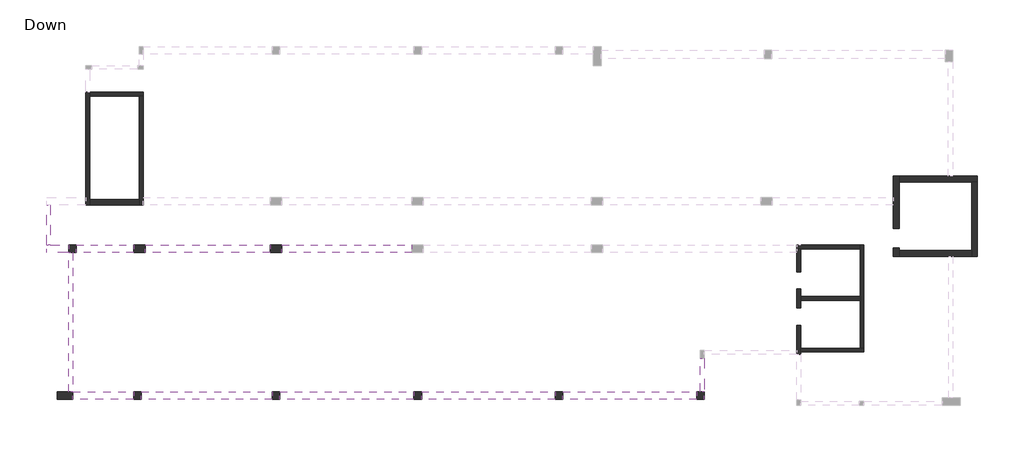
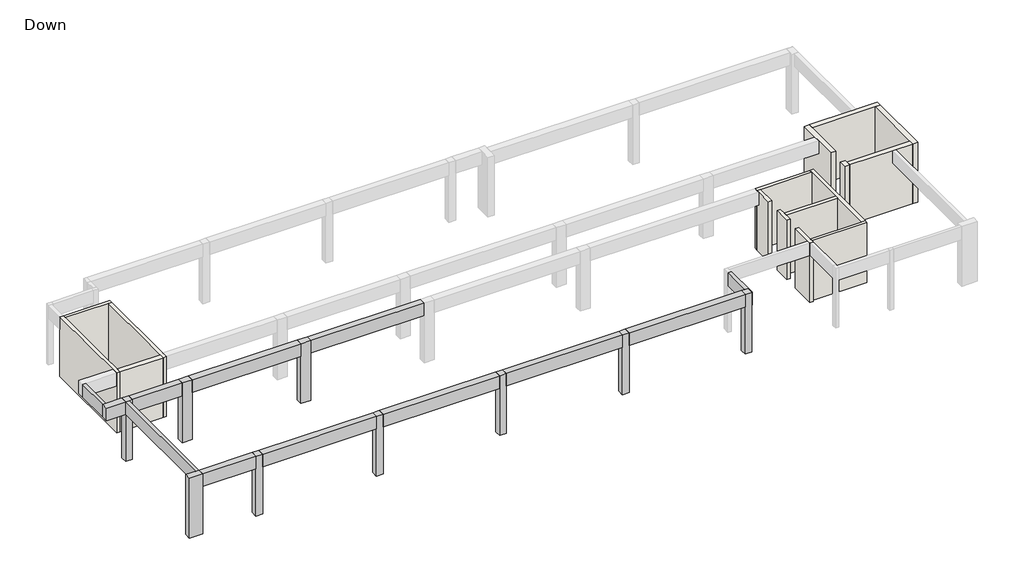
# One storey, part 1 of 2: 16 walls, 12 beams, 9 columns.
"""IFC4 building model written with IfcOpenShell, lengths in millimetres."""

from ifc_helpers import new_model, si_unit, frame, origin, origin_with_axes, place, context, project, spatial, polyline, outline, extrude, faceted_brep, element, save

model = new_model("IFC4")

# Units and contexts
model_context = context("Model", 3, world=origin())
ifc_project = project(units=[si_unit("LENGTHUNIT", "METRE", prefix="MILLI")], contexts=[model_context])

# Site, building, storey
site = spatial("IfcSite", under=ifc_project)
building = spatial("IfcBuilding", under=site)
storey = spatial("IfcBuildingStorey", under=building, Name="Down", Elevation=0.0)

# Beams
placement = place(None, origin())
element("IfcBeam", 1, ObjectType="Concrete Rectengular Beam : 20/80", at=placement, inside=storey, context=model_context, shape_type="Brep", body=[
    faceted_brep([(15342.1345122, -9540.2012066, 3800.0), (15342.1345122, -9940.2012066, 3800.0), (15344.7363769, -9940.2012066, 3800.0), (15344.7363769, -7771.4322554, 3800.0), (15144.7363769, -7771.4322554, 3800.0), (15144.7363769, -9540.2012066, 3800.0), (15144.7363769, -7771.4322554, 3520.0), (15144.7363769, -7771.4322554, 3000.0), (15144.7363769, -9540.2012066, 3000.0), (15144.7363769, -9540.2012066, 3520.0), (15342.1345122, -9940.2012066, 3000.0), (15342.1345122, -9540.2012066, 3000.0), (15344.7363769, -7771.4322554, 3000.0), (15344.7363769, -9940.2012066, 3000.0)], [[[0, 1, 2, 3, 4, 5]], [[5, 4, 6, 7, 8, 9]], [[10, 11, 8, 7, 12, 13]], [[12, 3, 2, 13]], [[0, 11, 10, 1]], [[11, 0, 5, 9, 8]], [[4, 3, 12, 7, 6]], [[13, 2, 1, 10]]]),
])
element("IfcBeam", 2, ObjectType="Concrete Rectengular Beam : 20/80", at=placement, inside=storey, context=model_context, shape_type="Brep", body=[
    faceted_brep([(-17707.5957255, -2249.6811448, 3800.0), (-17907.5957255, -2249.6811448, 3800.0), (-17907.5957255, -9540.2012066, 3800.0), (-17707.5957255, -9540.2012066, 3800.0), (-17907.5957255, -2249.6811448, 3000.0), (-17907.5957255, -9540.2012066, 3000.0), (-17707.5957255, -2249.6811448, 3000.0), (-17707.5957255, -9540.2012066, 3000.0), (-17707.5957255, -2249.6811448, 3520.0), (-17707.5957255, -9540.2012066, 3520.0)], [[[0, 1, 2, 3]], [[1, 4, 5, 2]], [[4, 6, 7, 5]], [[6, 8, 0, 3, 9, 7]], [[1, 0, 8, 6, 4]], [[3, 2, 5, 7, 9]]]),
])
element("IfcBeam", 3, ObjectType="Concrete Rectengular Beam : 20/80", at=placement, inside=storey, context=model_context, shape_type="Brep", body=[
    faceted_brep([(-18867.5920656, 245.3255739, 3800.0), (-19067.5920656, 245.3255739, 3800.0), (-19067.5920656, -1849.6811448, 3800.0), (-18867.5920656, -1849.6811448, 3800.0), (-18867.5920656, 245.3255739, 3000.0), (-18867.5920656, 245.3255739, 3520.0), (-18867.5920656, -1849.6811448, 3520.0), (-18867.5920656, -1849.6811448, 3000.0), (-19067.5920656, 245.3255739, 3000.0), (-19067.5920656, -1849.6811448, 3000.0)], [[[0, 1, 2, 3]], [[4, 5, 0, 3, 6, 7]], [[8, 4, 7, 9]], [[1, 8, 9, 2]], [[1, 0, 5, 4, 8]], [[3, 2, 9, 7, 6]]]),
])
element("IfcBeam", 4, ObjectType="Concrete Rectengular Beam : 40/80", at=placement, inside=storey, context=model_context, shape_type="SweptSolid", body=[
    extrude(outline(polyline([(7948.8072182, -9940.2012066), (7948.8072182, -9540.2012066), (14942.1345122, -9540.2012066), (14942.1345122, -9940.2012066), (7948.8072182, -9940.2012066)])), frame((0.0, 0.0, 3000.0), z_axis=(0.0, 0.0, 1.0), x_axis=(1.0, 0.0, 0.0)), (0.0, 0.0, 1.0), 800.0),
])
element("IfcBeam", 5, ObjectType="Concrete Rectengular Beam : 40/80", at=placement, inside=storey, context=model_context, shape_type="SweptSolid", body=[
    extrude(outline(polyline([(551.39348, -9940.2012066), (551.39348, -9540.2012066), (7548.8072182, -9540.2012066), (7548.8072182, -9940.2012066), (551.39348, -9940.2012066)])), frame((0.0, 0.0, 3000.0), z_axis=(0.0, 0.0, 1.0), x_axis=(1.0, 0.0, 0.0)), (0.0, 0.0, 1.0), 800.0),
])
element("IfcBeam", 6, ObjectType="Concrete Rectengular Beam : 40/80", at=placement, inside=storey, context=model_context, shape_type="SweptSolid", body=[
    extrude(outline(polyline([(-6857.9830653, -9940.2012066), (-6857.9830653, -9540.2012066), (151.39348, -9540.2012066), (151.39348, -9940.2012066), (-6857.9830653, -9940.2012066)])), frame((0.0, 0.0, 3000.0), z_axis=(0.0, 0.0, 1.0), x_axis=(1.0, 0.0, 0.0)), (0.0, 0.0, 1.0), 800.0),
])
element("IfcBeam", 7, ObjectType="Concrete Rectengular Beam : 40/80", at=placement, inside=storey, context=model_context, shape_type="SweptSolid", body=[
    extrude(outline(polyline([(-14112.2396142, -9940.2012066), (-14112.2396142, -9540.2012066), (-7257.9830653, -9540.2012066), (-7257.9830653, -9940.2012066), (-14112.2396142, -9940.2012066)])), frame((0.0, 0.0, 3000.0), z_axis=(0.0, 0.0, 1.0), x_axis=(1.0, 0.0, 0.0)), (0.0, 0.0, 1.0), 800.0),
])
element("IfcBeam", 8, ObjectType="Concrete Rectengular Beam : 40/80", at=placement, inside=storey, context=model_context, shape_type="Brep", body=[
    faceted_brep([(-14512.2396142, -9940.2012066, 3800.0), (-14512.2396142, -9540.2012066, 3800.0), (-17707.5957255, -9540.2012066, 3800.0), (-17707.5957255, -9940.2012066, 3800.0), (-14512.2396142, -9540.2012066, 3000.0), (-17707.5957255, -9540.2012066, 3000.0), (-17707.5957255, -9540.2012066, 3520.0), (-14512.2396142, -9940.2012066, 3000.0), (-17707.5957255, -9940.2012066, 3000.0)], [[[0, 1, 2, 3]], [[1, 4, 5, 6, 2]], [[4, 7, 8, 5]], [[7, 0, 3, 8]], [[1, 0, 7, 4]], [[3, 2, 6, 5, 8]]]),
])
element("IfcBeam", 9, ObjectType="Concrete Rectengular Beam : 40/80", at=placement, inside=storey, context=model_context, shape_type="SweptSolid", body=[
    extrude(outline(polyline([(-2249.6811448, 3000.0), (-2249.6811448, 3800.0), (-1851.1339506, 3800.0), (-1851.1339506, 3520.0), (-1849.6811448, 3520.0), (-1849.6811448, 3000.0), (-2249.6811448, 3000.0)])), frame((-17507.5957255, 0.0, 0.0), z_axis=(1.0, 0.0, 0.0), x_axis=(0.0, 1.0, 0.0)), (0.0, 0.0, 1.0), 2997.9865781),
])
element("IfcBeam", 10, ObjectType="Concrete Rectengular Beam : 40/80", at=placement, inside=storey, context=model_context, shape_type="SweptSolid", body=[
    extrude(outline(polyline([(-2249.6811448, 3000.0), (-2249.6811448, 3800.0), (-1851.1339506, 3800.0), (-1851.1339506, 3520.0), (-1849.6811448, 3520.0), (-1849.6811448, 3000.0), (-2249.6811448, 3000.0)])), frame((-13909.6091474, 0.0, 0.0), z_axis=(1.0, 0.0, 0.0), x_axis=(0.0, 1.0, 0.0)), (0.0, 0.0, 1.0), 6551.6260822),
])
element("IfcBeam", 11, ObjectType="Concrete Rectengular Beam : 40/80", at=placement, inside=storey, context=model_context, shape_type="SweptSolid", body=[
    extrude(outline(polyline([(-2249.6811448, 3000.0), (-2249.6811448, 3800.0), (-1851.1339506, 3800.0), (-1851.1339506, 3520.0), (-1849.6811448, 3520.0), (-1849.6811448, 3000.0), (-2249.6811448, 3000.0)])), frame((-6757.9830653, 0.0, 0.0), z_axis=(1.0, 0.0, 0.0), x_axis=(0.0, 1.0, 0.0)), (0.0, 0.0, 1.0), 6809.3765453),
])
element("IfcBeam", 12, ObjectType="Concrete Rectengular Beam : 40/80", at=placement, inside=storey, context=model_context, shape_type="Brep", body=[
    faceted_brep([(-19067.5920656, -1849.6811448, 3800.0), (-19067.5920656, -2249.6811448, 3800.0), (-17907.5957255, -2249.6811448, 3800.0), (-17907.5957255, -1851.1339506, 3800.0), (-18867.5920656, -1851.1339506, 3800.0), (-18867.5920656, -1849.6811448, 3800.0), (-19067.5920656, -1849.6811448, 3000.0), (-18867.5920656, -1849.6811448, 3520.0), (-17907.5957255, -1849.6811448, 3520.0), (-17907.5957255, -1849.6811448, 3000.0), (-18867.5920656, -1849.6811448, 3000.0), (-17907.5957255, -2249.6811448, 3000.0), (-19067.5920656, -2249.6811448, 3000.0), (-17907.5957255, -1851.1339506, 3520.0), (-18867.5920656, -1851.1339506, 3520.0)], [[[0, 1, 2, 3, 4, 5]], [[6, 0, 5, 7, 8, 9, 10]], [[9, 11, 12, 6, 10]], [[11, 2, 1, 12]], [[2, 11, 9, 8, 13, 3]], [[1, 0, 6, 12]], [[7, 14, 13, 8]], [[14, 4, 3, 13]], [[4, 14, 7, 5]]]),
])

# Columns
element("IfcColumn", 13, ObjectType="Concrete Rectengular Column : 40/40", at=placement, inside=storey, context=model_context, shape_type="Brep", body=[
    faceted_brep([(-17507.5957255, -1849.6811448, 0.0), (-17507.5957255, -2249.6811448, 0.0), (-17907.5957255, -2249.6811448, 0.0), (-17907.5957255, -1849.6811448, 0.0), (-17507.5957255, -1849.6811448, 3800.0), (-17507.5957255, -1851.1339506, 3800.0), (-17507.5957255, -2249.6811448, 3800.0), (-17507.5957255, -1849.6811448, 3520.0), (-17707.5957255, -2249.6811448, 3800.0), (-17907.5957255, -2249.6811448, 3800.0), (-17907.5957255, -1851.1339506, 3800.0), (-17907.5957255, -1849.6811448, 3800.0), (-17907.5957255, -1849.6811448, 3520.0)], [[[0, 1, 2, 3]], [[4, 5, 6, 1, 0, 7]], [[6, 8, 9, 2, 1]], [[9, 10, 11, 12, 3, 2]], [[11, 4, 7, 0, 3, 12]], [[4, 11, 10, 9, 8, 6, 5]]]),
])
element("IfcColumn", 14, ObjectType="Concrete Rectengular Column : 40/40", at=placement, inside=storey, context=model_context, shape_type="SweptSolid", body=[
    extrude(outline(polyline([(-14112.2396142, -9540.2012066), (-14112.2396142, -9940.2012066), (-14512.2396142, -9940.2012066), (-14512.2396142, -9540.2012066), (-14112.2396142, -9540.2012066)])), origin_with_axes(), (0.0, 0.0, 1.0), 3800.0),
])
element("IfcColumn", 15, ObjectType="Concrete Rectengular Column : 40/40", at=placement, inside=storey, context=model_context, shape_type="SweptSolid", body=[
    extrude(outline(polyline([(-6857.9830653, -9540.2012066), (-6857.9830653, -9940.2012066), (-7257.9830653, -9940.2012066), (-7257.9830653, -9540.2012066), (-6857.9830653, -9540.2012066)])), origin_with_axes(), (0.0, 0.0, 1.0), 3800.0),
])
element("IfcColumn", 16, ObjectType="Concrete Rectengular Column : 40/40", at=placement, inside=storey, context=model_context, shape_type="SweptSolid", body=[
    extrude(outline(polyline([(551.39348, -9540.2012066), (551.39348, -9940.2012066), (151.39348, -9940.2012066), (151.39348, -9540.2012066), (551.39348, -9540.2012066)])), origin_with_axes(), (0.0, 0.0, 1.0), 3800.0),
])
element("IfcColumn", 17, ObjectType="Concrete Rectengular Column : 40/40", at=placement, inside=storey, context=model_context, shape_type="SweptSolid", body=[
    extrude(outline(polyline([(7948.8072182, -9540.2012066), (7948.8072182, -9940.2012066), (7548.8072182, -9940.2012066), (7548.8072182, -9540.2012066), (7948.8072182, -9540.2012066)])), origin_with_axes(), (0.0, 0.0, 1.0), 3800.0),
])
element("IfcColumn", 18, ObjectType="Concrete Rectengular Column : 40/40", at=placement, inside=storey, context=model_context, shape_type="Brep", body=[
    faceted_brep([(15342.1345122, -9540.2012066, 0.0), (15342.1345122, -9940.2012066, 0.0), (14942.1345122, -9940.2012066, 0.0), (14942.1345122, -9540.2012066, 0.0), (15342.1345122, -9540.2012066, 3800.0), (15342.1345122, -9940.2012066, 3800.0), (14942.1345122, -9940.2012066, 3800.0), (14942.1345122, -9540.2012066, 3800.0), (15144.7363769, -9540.2012066, 3800.0)], [[[0, 1, 2, 3]], [[4, 5, 1, 0]], [[5, 6, 2, 1]], [[6, 7, 3, 2]], [[7, 8, 4, 0, 3]], [[4, 8, 7, 6, 5]]]),
])
element("IfcColumn", 19, ObjectType="Concrete Rectengular Column : 40/60", at=placement, inside=storey, context=model_context, shape_type="Brep", body=[
    faceted_brep([(-14509.6091474, -1849.6811448, 0.0), (-13909.6091474, -1849.6811448, 0.0), (-13909.6091474, -2249.6811448, 0.0), (-14509.6091474, -2249.6811448, 0.0), (-14509.6091474, -1849.6811448, 3800.0), (-13909.6091474, -1849.6811448, 3800.0), (-13909.6091474, -1849.6811448, 3520.0), (-14509.6091474, -1849.6811448, 3520.0), (-13909.6091474, -1851.1339506, 3800.0), (-13909.6091474, -2249.6811448, 3800.0), (-14509.6091474, -2249.6811448, 3800.0), (-14509.6091474, -1851.1339506, 3800.0)], [[[0, 1, 2, 3]], [[4, 5, 6, 1, 0, 7]], [[5, 8, 9, 2, 1, 6]], [[9, 10, 3, 2]], [[10, 11, 4, 7, 0, 3]], [[4, 11, 10, 9, 8, 5]]]),
])
element("IfcColumn", 20, ObjectType="Concrete Rectengular Column : 40/60", at=placement, inside=storey, context=model_context, shape_type="Brep", body=[
    faceted_brep([(-7357.9830653, -1849.6811448, 0.0), (-6757.9830653, -1849.6811448, 0.0), (-6757.9830653, -2249.6811448, 0.0), (-7357.9830653, -2249.6811448, 0.0), (-7357.9830653, -1849.6811448, 3800.0), (-6757.9830653, -1849.6811448, 3800.0), (-6757.9830653, -1849.6811448, 3520.0), (-7357.9830653, -1849.6811448, 3520.0), (-6757.9830653, -1851.1339506, 3800.0), (-6757.9830653, -2249.6811448, 3800.0), (-7357.9830653, -2249.6811448, 3800.0), (-7357.9830653, -1851.1339506, 3800.0)], [[[0, 1, 2, 3]], [[4, 5, 6, 1, 0, 7]], [[5, 8, 9, 2, 1, 6]], [[9, 10, 3, 2]], [[10, 11, 4, 7, 0, 3]], [[4, 11, 10, 9, 8, 5]]]),
])
element("IfcColumn", 21, ObjectType="Concrete Rectengular Column : 40/80", at=placement, inside=storey, context=model_context, shape_type="SweptSolid", body=[
    extrude(outline(polyline([(-18507.5957255, -9540.2012066), (-17707.5957255, -9540.2012066), (-17707.5957255, -9940.2012066), (-18507.5957255, -9940.2012066), (-18507.5957255, -9540.2012066)])), origin_with_axes(), (0.0, 0.0, 1.0), 3800.0),
])

# Walls
element("IfcWall", 22, ObjectType="20", at=placement, inside=storey, context=model_context, shape_type="Brep", body=[
    faceted_brep([(20195.2300261, -6051.4322554, 0.0), (20195.2300261, -7571.4322554, 0.0), (20195.2300261, -7571.4322554, 3800.0), (20195.2300261, -7371.4322554, 3800.0), (20195.2300261, -6051.4322554, 3800.0), (20195.2300261, -6051.4322554, 3520.0), (20395.2300261, -6051.4322554, 0.0), (20395.2300261, -6051.4322554, 3800.0), (20395.2300261, -7251.1339506, 3800.0), (20395.2300261, -7451.1339506, 3800.0), (20395.2300261, -7571.4322554, 3800.0), (20395.2300261, -7571.4322554, 0.0), (20395.2300261, -7451.1339506, 0.0), (20395.2300261, -7251.1339506, 0.0)], [[[0, 1, 2, 3, 4, 5]], [[6, 7, 8, 9, 10, 11, 12, 13]], [[1, 0, 6, 13, 12, 11]], [[2, 1, 11, 10]], [[4, 3, 2, 10, 9, 8, 7]], [[0, 5, 4, 7, 6]]]),
])
element("IfcWall", 23, ObjectType="20", at=placement, inside=storey, context=model_context, shape_type="Brep", body=[
    faceted_brep([(20395.2300261, -7451.1339506, 0.0), (23696.3370418, -7451.1339506, 0.0), (23696.3370418, -7451.1339506, 3520.0), (23696.3370418, -7451.1339506, 3800.0), (20395.2300261, -7451.1339506, 3800.0), (20395.2300261, -7451.1339506, 3520.0), (20395.2300261, -7251.1339506, 0.0), (20395.2300261, -7251.1339506, 3800.0), (23496.3370418, -7251.1339506, 3800.0), (23696.3370418, -7251.1339506, 3800.0), (23696.3370418, -7251.1339506, 0.0), (23496.3370418, -7251.1339506, 0.0)], [[[0, 1, 2, 3, 4, 5]], [[6, 7, 8, 9, 10, 11]], [[1, 0, 6, 11, 10]], [[4, 3, 9, 8, 7]], [[0, 5, 4, 7, 6]], [[3, 2, 1, 10, 9]]]),
])
element("IfcWall", 24, ObjectType="20", at=placement, inside=storey, context=model_context, shape_type="Brep", body=[
    faceted_brep([(23696.3370418, -7251.1339506, 0.0), (23696.3370418, -1851.1339506, 0.0), (23696.3370418, -1851.1339506, 3520.0), (23696.3370418, -1851.1339506, 3800.0), (23696.3370418, -7251.1339506, 3800.0), (23496.3370418, -7251.1339506, 0.0), (23496.3370418, -7251.1339506, 3800.0), (23496.3370418, -4748.6834924, 3800.0), (23496.3370418, -4548.6834924, 3800.0), (23496.3370418, -2051.1339506, 3800.0), (23496.3370418, -1851.1339506, 3800.0), (23496.3370418, -1851.1339506, 0.0), (23496.3370418, -2051.1339506, 0.0), (23496.3370418, -4548.6834924, 0.0), (23496.3370418, -4748.6834924, 0.0)], [[[0, 1, 2, 3, 4]], [[5, 6, 7, 8, 9, 10, 11, 12, 13, 14]], [[1, 0, 5, 14, 13, 12, 11]], [[4, 3, 10, 9, 8, 7, 6]], [[0, 4, 6, 5]], [[3, 2, 1, 11, 10]]]),
])
element("IfcWall", 25, ObjectType="20", at=placement, inside=storey, context=model_context, shape_type="Brep", body=[
    faceted_brep([(23496.3370418, -1851.1339506, 0.0), (20196.3370418, -1851.1339506, 0.0), (20196.3370418, -1851.1339506, 3000.0), (20196.3370418, -1851.1339506, 3520.0), (20196.3370418, -1851.1339506, 3800.0), (23496.3370418, -1851.1339506, 3800.0), (23496.3370418, -2051.1339506, 0.0), (23496.3370418, -2051.1339506, 3800.0), (20396.3370418, -2051.1339506, 3800.0), (20196.3370418, -2051.1339506, 3800.0), (20196.3370418, -2051.1339506, 0.0), (20396.3370418, -2051.1339506, 0.0)], [[[0, 1, 2, 3, 4, 5]], [[6, 7, 8, 9, 10, 11]], [[1, 0, 6, 11, 10]], [[5, 4, 9, 8, 7]], [[0, 5, 7, 6]], [[4, 3, 2, 1, 10, 9]]]),
])
element("IfcWall", 26, ObjectType="20", at=placement, inside=storey, context=model_context, shape_type="Brep", body=[
    faceted_brep([(20196.3370418, -2051.1339506, 0.0), (20196.3370418, -3251.1339506, 0.0), (20196.3370418, -3251.1339506, 3520.0), (20196.3370418, -3251.1339506, 3800.0), (20196.3370418, -2249.6811448, 3800.0), (20196.3370418, -2051.1339506, 3800.0), (20396.3370418, -2051.1339506, 0.0), (20396.3370418, -2051.1339506, 3800.0), (20396.3370418, -3251.1339506, 3800.0), (20396.3370418, -3251.1339506, 3520.0), (20396.3370418, -3251.1339506, 0.0)], [[[0, 1, 2, 3, 4, 5]], [[6, 7, 8, 9, 10]], [[1, 0, 6, 10]], [[3, 2, 1, 10, 9, 8]], [[5, 4, 3, 8, 7]], [[0, 5, 7, 6]]]),
])
element("IfcWall", 27, ObjectType="20", at=placement, inside=storey, context=model_context, shape_type="Brep", body=[
    faceted_brep([(20196.3370418, -4150.7725523, 0.0), (20196.3370418, -5149.7829976, 0.0), (20196.3370418, -5149.7829976, 3520.0), (20196.3370418, -5149.7829976, 3800.0), (20196.3370418, -4150.7725523, 3800.0), (20196.3370418, -4150.7725523, 3520.0), (20396.3370418, -4150.7725523, 0.0), (20396.3370418, -4150.7725523, 3520.0), (20396.3370418, -4150.7725523, 3800.0), (20396.3370418, -4548.6834924, 3800.0), (20396.3370418, -4748.6834924, 3800.0), (20396.3370418, -5149.7829976, 3800.0), (20396.3370418, -5149.7829976, 3520.0), (20396.3370418, -5149.7829976, 0.0), (20396.3370418, -4748.6834924, 0.0), (20396.3370418, -4548.6834924, 0.0)], [[[0, 1, 2, 3, 4, 5]], [[6, 7, 8, 9, 10, 11, 12, 13, 14, 15]], [[1, 0, 6, 15, 14, 13]], [[3, 2, 1, 13, 12, 11]], [[4, 3, 11, 10, 9, 8]], [[0, 5, 4, 8, 7, 6]]]),
])
element("IfcWall", 28, ObjectType="20", at=placement, inside=storey, context=model_context, shape_type="SweptSolid", body=[
    extrude(outline(polyline([(23496.3370418, -4748.6834924), (20396.3370418, -4748.6834924), (20396.3370418, -4548.6834924), (23496.3370418, -4548.6834924), (23496.3370418, -4748.6834924)])), origin_with_axes(), (0.0, 0.0, 1.0), 3800.0),
])
element("IfcWall", 29, ObjectType="20", at=placement, inside=storey, context=model_context, shape_type="Brep", body=[
    faceted_brep([(-16809.1027603, 245.3255739, 0.0), (-16809.1027603, 545.3255739, 0.0), (-16809.1027603, 5957.8562202, 0.0), (-16809.1027603, 6157.8562202, 0.0), (-16809.1027603, 6157.8562202, 3000.0), (-16809.1027603, 6157.8562202, 3800.0), (-16809.1027603, 5957.8562202, 3800.0), (-16809.1027603, 1758.6282173, 3800.0), (-16809.1027603, 545.3255739, 3800.0), (-16809.1027603, 245.3255739, 3800.0), (-17009.1027603, 245.3255739, 0.0), (-17009.1027603, 245.3255739, 3800.0), (-17009.1027603, 6157.8562202, 3800.0), (-17009.1027603, 6157.8562202, 3000.0), (-17009.1027603, 6157.8562202, 0.0)], [[[0, 1, 2, 3, 4, 5, 6, 7, 8, 9]], [[10, 11, 12, 13, 14]], [[3, 2, 1, 0, 10, 14]], [[9, 8, 7, 6, 5, 12, 11]], [[5, 4, 3, 14, 13, 12]], [[0, 9, 11, 10]]]),
])
element("IfcWall", 30, ObjectType="20", at=placement, inside=storey, context=model_context, shape_type="Brep", body=[
    faceted_brep([(-16809.1027603, 5957.8562202, 0.0), (-14212.0714244, 5957.8562202, 0.0), (-14012.0714244, 5957.8562202, 0.0), (-14012.0714244, 5957.8562202, 3800.0), (-14212.0714244, 5957.8562202, 3800.0), (-16809.1027603, 5957.8562202, 3800.0), (-16809.1027603, 6157.8562202, 0.0), (-16809.1027603, 6157.8562202, 3520.0), (-16809.1027603, 6157.8562202, 3800.0), (-14012.0714244, 6157.8562202, 3800.0), (-14012.0714244, 6157.8562202, 3520.0), (-14012.0714244, 6157.8562202, 0.0)], [[[0, 1, 2, 3, 4, 5]], [[6, 7, 8, 9, 10, 11]], [[2, 1, 0, 6, 11]], [[5, 4, 3, 9, 8]], [[0, 5, 8, 7, 6]], [[3, 2, 11, 10, 9]]]),
])
element("IfcWall", 31, ObjectType="20", at=placement, inside=storey, context=model_context, shape_type="Brep", body=[
    faceted_brep([(-14212.0714244, 5957.8562202, 0.0), (-14212.0714244, 545.3255739, 0.0), (-14212.0714244, 245.3255739, 0.0), (-14212.0714244, 245.3255739, 3800.0), (-14212.0714244, 545.3255739, 3800.0), (-14212.0714244, 1758.6282173, 3800.0), (-14212.0714244, 5957.8562202, 3800.0), (-14012.0714244, 5957.8562202, 0.0), (-14012.0714244, 5957.8562202, 3800.0), (-14012.0714244, 645.3255739, 3800.0), (-14012.0714244, 245.3255739, 3800.0), (-14012.0714244, 245.3255739, 0.0)], [[[0, 1, 2, 3, 4, 5, 6]], [[7, 8, 9, 10, 11]], [[2, 1, 0, 7, 11]], [[6, 5, 4, 3, 10, 9, 8]], [[0, 6, 8, 7]], [[3, 2, 11, 10]]]),
])
element("IfcWall", 32, ObjectType="30", at=placement, inside=storey, context=model_context, shape_type="Brep", body=[
    faceted_brep([(25541.4195047, -992.8836023, 0.0), (25541.4195047, 1458.6282173, 0.0), (25541.4195047, 1758.6282173, 0.0), (25541.4195047, 1758.6282173, 3800.0), (25541.4195047, 1458.6282173, 3800.0), (25541.4195047, -992.8836023, 3800.0), (25541.4195047, -992.8836023, 3600.0), (25241.4195047, -992.8836023, 0.0), (25241.4195047, -992.8836023, 3520.0), (25241.4195047, -992.8836023, 3800.0), (25241.4195047, 245.3255739, 3800.0), (25241.4195047, 645.3255739, 3800.0), (25241.4195047, 1758.6282173, 3800.0), (25241.4195047, 1758.6282173, 3520.0), (25241.4195047, 1758.6282173, 0.0), (25540.6606912, -992.8836023, 3800.0)], [[[0, 1, 2, 3, 4, 5, 6]], [[7, 8, 9, 10, 11, 12, 13, 14]], [[2, 1, 0, 7, 14]], [[5, 4, 3, 12, 11, 10, 9, 15]], [[0, 6, 5, 15, 9, 8, 7]], [[3, 2, 14, 13, 12]]]),
])
element("IfcWall", 33, ObjectType="30", at=placement, inside=storey, context=model_context, shape_type="Brep", body=[
    faceted_brep([(25541.4195047, 1458.6282173, 0.0), (29339.6053211, 1458.6282173, 0.0), (29639.6053211, 1458.6282173, 0.0), (29639.6053211, 1458.6282173, 3800.0), (29339.6053211, 1458.6282173, 3800.0), (25541.4195047, 1458.6282173, 3800.0), (25541.4195047, 1458.6282173, 3600.0), (25541.4195047, 1758.6282173, 0.0), (25541.4195047, 1758.6282173, 3800.0), (28101.2236194, 1758.6282173, 3800.0), (29639.6053211, 1758.6282173, 3800.0), (29639.6053211, 1758.6282173, 0.0)], [[[0, 1, 2, 3, 4, 5, 6]], [[7, 8, 9, 10, 11]], [[2, 1, 0, 7, 11]], [[5, 4, 3, 10, 9, 8]], [[0, 6, 5, 8, 7]], [[3, 2, 11, 10]]]),
])
element("IfcWall", 34, ObjectType="30", at=placement, inside=storey, context=model_context, shape_type="Brep", body=[
    faceted_brep([(29339.6053211, 1458.6282173, 0.0), (29339.6053211, -2141.3717827, 0.0), (29339.6053211, -2441.3717827, 0.0), (29339.6053211, -2441.3717827, 3800.0), (29339.6053211, -2141.3717827, 3800.0), (29339.6053211, 1458.6282173, 3800.0), (29339.6053211, 1458.6282173, 3600.0), (29639.6053211, 1458.6282173, 0.0), (29639.6053211, 1458.6282173, 3800.0), (29639.6053211, -2441.3717827, 3800.0), (29639.6053211, -2441.3717827, 0.0)], [[[0, 1, 2, 3, 4, 5, 6]], [[7, 8, 9, 10]], [[2, 1, 0, 7, 10]], [[5, 4, 3, 9, 8]], [[0, 6, 5, 8, 7]], [[3, 2, 10, 9]]]),
])
element("IfcWall", 35, ObjectType="30", at=placement, inside=storey, context=model_context, shape_type="Brep", body=[
    faceted_brep([(29339.6053211, -2141.3717827, 0.0), (25540.6606912, -2141.3717827, 0.0), (25540.6606912, -2141.3717827, 3600.0), (25540.6606912, -2141.3717827, 3800.0), (29339.6053211, -2141.3717827, 3800.0), (29339.6053211, -2141.3717827, 3600.0), (29339.6053211, -2441.3717827, 0.0), (29339.6053211, -2441.3717827, 3800.0), (28136.856558, -2441.3717827, 3800.0), (25540.6606912, -2441.3717827, 3800.0), (25540.6606912, -2441.3717827, 0.0)], [[[0, 1, 2, 3, 4, 5]], [[6, 7, 8, 9, 10]], [[1, 0, 6, 10]], [[4, 3, 9, 8, 7]], [[0, 5, 4, 7, 6]], [[3, 2, 1, 10, 9]]]),
])
element("IfcWall", 36, ObjectType="30", at=placement, inside=storey, context=model_context, shape_type="Brep", body=[
    faceted_brep([(25540.6606912, -2441.3717827, 0.0), (25540.6606912, -2141.3717827, 0.0), (25540.6606912, -1996.3717827, 0.0), (25540.6606912, -1996.3717827, 3520.0), (25540.6606912, -1996.3717827, 3800.0), (25540.6606912, -2141.3717827, 3800.0), (25540.6606912, -2441.3717827, 3800.0), (25240.6606912, -2441.3717827, 0.0), (25240.6606912, -2441.3717827, 3520.0), (25240.6606912, -2441.3717827, 3800.0), (25240.6606912, -1996.3717827, 3800.0), (25240.6606912, -1996.3717827, 3520.0), (25240.6606912, -1996.3717827, 0.0), (25241.4195047, -1996.3717827, 3800.0)], [[[0, 1, 2, 3, 4, 5, 6]], [[7, 8, 9, 10, 11, 12]], [[2, 1, 0, 7, 12]], [[4, 3, 2, 12, 11, 10, 13]], [[6, 5, 4, 13, 10, 9]], [[0, 6, 9, 8, 7]]]),
])
element("IfcWall", 37, ObjectType="30", at=placement, inside=storey, context=model_context, shape_type="Brep", body=[
    faceted_brep([(-14212.0714244, 545.3255739, 0.0), (-16809.1027603, 545.3255739, 0.0), (-16809.1027603, 545.3255739, 3600.0), (-16809.1027603, 545.3255739, 3800.0), (-14212.0714244, 545.3255739, 3800.0), (-14212.0714244, 545.3255739, 3600.0), (-14212.0714244, 245.3255739, 0.0), (-14212.0714244, 245.3255739, 3800.0), (-16809.1027603, 245.3255739, 3800.0), (-16809.1027603, 245.3255739, 0.0)], [[[0, 1, 2, 3, 4, 5]], [[6, 7, 8, 9]], [[1, 0, 6, 9]], [[4, 3, 8, 7]], [[0, 5, 4, 7, 6]], [[3, 2, 1, 9, 8]]]),
])

save(model, "model.ifc")

# Revit data of these elements
# Project information
#   Project Issue Date = "Issue Date"
#   Project Status = "Project Status"
#   Client Name = "לקוח"
#   Project Address = "Enter address here"
#   Project Name = "Project 041"
#   Project Number = "מספר פרויקט"
# Type "Concrete Rectengular Beam : 20/80"
#   Length [instance default] = 152.4 cm
#   b = 20 cm
#   h = 80 cm
#   Structural Material [instance default] = Concrete
#   Assembly Code = ""
# Type "Concrete Rectengular Beam : 40/80"
#   Length [instance default] = 152.4 cm
#   b = 40 cm
#   h = 80 cm
#   Structural Material [instance default] = Concrete
#   Assembly Code = ""
# Type "Concrete Rectengular Column : 40/40"
#   b = 40 cm
#   h = 40 cm
#   Structural Material [instance default] = Concrete
# Type "Concrete Rectengular Column : 40/60"
#   b = 40 cm
#   h = 60 cm
#   Structural Material [instance default] = Concrete
# Type "Concrete Rectengular Column : 40/80"
#   b = 40 cm
#   h = 80 cm
#   Structural Material [instance default] = Concrete
# Type "20"
#   Layers, outside or top first: 20 cm "Concrete" (function 1)
# Type "30"
#   Layers, outside or top first: 30 cm "Concrete" (function 1)
# Element 1 (IfcBeam, "Concrete Rectengular Beam : 20/80")
#   Comments = ""
#   Mark = "B8"
#   SOFiSTiK_AMG_Comments = ""
#   SOFiSTiK_AMG_Scheduled = yes
#   SOFiSTiK_AMG_Adjusted = yes
#   Structural Material = Concrete
#   Phase Created = New Construction
#   Materials on its faces: "Concrete"
# Element 2 (IfcBeam, "Concrete Rectengular Beam : 20/80")
#   Comments = ""
#   Mark = "B9"
#   SOFiSTiK_AMG_Comments = ""
#   SOFiSTiK_AMG_Scheduled = yes
#   SOFiSTiK_AMG_Adjusted = yes
#   Structural Material = Concrete
#   Phase Created = New Construction
#   Materials on its faces: "Concrete"
# Element 3 (IfcBeam, "Concrete Rectengular Beam : 20/80")
#   Comments = ""
#   Mark = "B10"
#   SOFiSTiK_AMG_Comments = ""
#   SOFiSTiK_AMG_Scheduled = yes
#   SOFiSTiK_AMG_Adjusted = yes
#   Structural Material = Concrete
#   Phase Created = New Construction
#   Materials on its faces: "Concrete"
# Element 4 (IfcBeam, "Concrete Rectengular Beam : 40/80")
#   Comments = ""
#   Mark = "B17"
#   SOFiSTiK_AMG_Comments = ""
#   SOFiSTiK_AMG_Scheduled = yes
#   SOFiSTiK_AMG_Adjusted = yes
#   Structural Material = Concrete
#   Phase Created = New Construction
#   Materials on its faces: "Concrete"
# Element 5 (IfcBeam, "Concrete Rectengular Beam : 40/80")
#   Comments = ""
#   Mark = "B18"
#   SOFiSTiK_AMG_Comments = ""
#   SOFiSTiK_AMG_Scheduled = yes
#   SOFiSTiK_AMG_Adjusted = yes
#   Structural Material = Concrete
#   Phase Created = New Construction
#   Materials on its faces: "Concrete"
# Element 6 (IfcBeam, "Concrete Rectengular Beam : 40/80")
#   Comments = ""
#   Mark = "B19"
#   SOFiSTiK_AMG_Comments = ""
#   SOFiSTiK_AMG_Scheduled = yes
#   SOFiSTiK_AMG_Adjusted = yes
#   Structural Material = Concrete
#   Phase Created = New Construction
#   Materials on its faces: "Concrete"
# Element 7 (IfcBeam, "Concrete Rectengular Beam : 40/80")
#   Comments = ""
#   Mark = "B20"
#   SOFiSTiK_AMG_Comments = ""
#   SOFiSTiK_AMG_Scheduled = yes
#   SOFiSTiK_AMG_Adjusted = yes
#   Structural Material = Concrete
#   Phase Created = New Construction
#   Materials on its faces: "Concrete"
# Element 8 (IfcBeam, "Concrete Rectengular Beam : 40/80")
#   Comments = ""
#   Mark = "B21"
#   SOFiSTiK_AMG_Comments = ""
#   SOFiSTiK_AMG_Scheduled = yes
#   SOFiSTiK_AMG_Adjusted = yes
#   Structural Material = Concrete
#   Phase Created = New Construction
#   Materials on its faces: "Concrete"
# Element 9 (IfcBeam, "Concrete Rectengular Beam : 40/80")
#   Comments = ""
#   Mark = "B22"
#   SOFiSTiK_AMG_Comments = ""
#   SOFiSTiK_AMG_Scheduled = yes
#   SOFiSTiK_AMG_Adjusted = yes
#   Structural Material = Concrete
#   Phase Created = New Construction
#   Materials on its faces: "Concrete"
# Element 10 (IfcBeam, "Concrete Rectengular Beam : 40/80")
#   Comments = ""
#   Mark = "B23"
#   SOFiSTiK_AMG_Comments = ""
#   SOFiSTiK_AMG_Scheduled = yes
#   SOFiSTiK_AMG_Adjusted = yes
#   Structural Material = Concrete
#   Phase Created = New Construction
#   Materials on its faces: "Concrete"
# Element 11 (IfcBeam, "Concrete Rectengular Beam : 40/80")
#   Comments = ""
#   Mark = "B24"
#   SOFiSTiK_AMG_Comments = ""
#   SOFiSTiK_AMG_Scheduled = yes
#   SOFiSTiK_AMG_Adjusted = yes
#   Structural Material = Concrete
#   Phase Created = New Construction
#   Materials on its faces: "Concrete"
# Element 12 (IfcBeam, "Concrete Rectengular Beam : 40/80")
#   Comments = ""
#   Mark = "B33"
#   SOFiSTiK_AMG_Comments = ""
#   SOFiSTiK_AMG_Scheduled = yes
#   SOFiSTiK_AMG_Adjusted = yes
#   Structural Material = Concrete
#   Phase Created = New Construction
#   Materials on its faces: "Concrete"
# Element 13 (IfcColumn, "Concrete Rectengular Column : 40/40")
#   Comments = ""
#   Mark = "C8"
#   SOFiSTiK_AMG_Comments = ""
#   SOFiSTiK_AMG_Scheduled = yes
#   SOFiSTiK_AMG_Adjusted = yes
#   Structural Material = Concrete
#   Phase Created = New Construction
#   Materials on its faces: "Concrete"
# Element 14 (IfcColumn, "Concrete Rectengular Column : 40/40")
#   Comments = ""
#   Mark = "C9"
#   SOFiSTiK_AMG_Comments = ""
#   SOFiSTiK_AMG_Scheduled = yes
#   SOFiSTiK_AMG_Adjusted = yes
#   Structural Material = Concrete
#   Phase Created = New Construction
#   Materials on its faces: "Concrete"
# Element 15 (IfcColumn, "Concrete Rectengular Column : 40/40")
#   Comments = ""
#   Mark = "C10"
#   SOFiSTiK_AMG_Comments = ""
#   SOFiSTiK_AMG_Scheduled = yes
#   SOFiSTiK_AMG_Adjusted = yes
#   Structural Material = Concrete
#   Phase Created = New Construction
#   Materials on its faces: "Concrete"
# Element 16 (IfcColumn, "Concrete Rectengular Column : 40/40")
#   Comments = ""
#   Mark = "C11"
#   SOFiSTiK_AMG_Comments = ""
#   SOFiSTiK_AMG_Scheduled = yes
#   SOFiSTiK_AMG_Adjusted = yes
#   Structural Material = Concrete
#   Phase Created = New Construction
#   Materials on its faces: "Concrete"
# Element 17 (IfcColumn, "Concrete Rectengular Column : 40/40")
#   Comments = ""
#   Mark = "C12"
#   SOFiSTiK_AMG_Comments = ""
#   SOFiSTiK_AMG_Scheduled = yes
#   SOFiSTiK_AMG_Adjusted = yes
#   Structural Material = Concrete
#   Phase Created = New Construction
#   Materials on its faces: "Concrete"
# Element 18 (IfcColumn, "Concrete Rectengular Column : 40/40")
#   Comments = ""
#   Mark = "C13"
#   SOFiSTiK_AMG_Comments = ""
#   SOFiSTiK_AMG_Scheduled = yes
#   SOFiSTiK_AMG_Adjusted = yes
#   Structural Material = Concrete
#   Phase Created = New Construction
#   Materials on its faces: "Concrete"
# Element 19 (IfcColumn, "Concrete Rectengular Column : 40/60")
#   Comments = ""
#   Mark = "C18"
#   SOFiSTiK_AMG_Comments = ""
#   SOFiSTiK_AMG_Scheduled = yes
#   SOFiSTiK_AMG_Adjusted = yes
#   Structural Material = Concrete
#   Phase Created = New Construction
#   Materials on its faces: "Concrete"
# Element 20 (IfcColumn, "Concrete Rectengular Column : 40/60")
#   Comments = ""
#   Mark = "C19"
#   SOFiSTiK_AMG_Comments = ""
#   SOFiSTiK_AMG_Scheduled = yes
#   SOFiSTiK_AMG_Adjusted = yes
#   Structural Material = Concrete
#   Phase Created = New Construction
#   Materials on its faces: "Concrete"
# Element 21 (IfcColumn, "Concrete Rectengular Column : 40/80")
#   Comments = ""
#   Mark = "C27"
#   SOFiSTiK_AMG_Comments = ""
#   SOFiSTiK_AMG_Scheduled = yes
#   SOFiSTiK_AMG_Adjusted = yes
#   Structural Material = Concrete
#   Phase Created = New Construction
#   Materials on its faces: "Concrete"
# Element 22 (IfcWall, "20")
#   Comments = ""
#   Mark = "W7"
#   SOFiSTiK_EdgeZones = "W7"
#   SOFiSTiK_AMG_Comments = ""
#   Top Offset = 0 cm
#   Base Offset = 0 cm
#   wall height = 380 cm
#   SOFiSTiK_AMG_Scheduled = yes
#   SOFiSTiK_AMG_Adjusted = yes
#   Phase Created = New Construction
#   Base Constraint = Down
#   Top Constraint = Typical Floor
#   Materials on its faces: "Concrete"
# Element 23 (IfcWall, "20")
#   Comments = ""
#   Mark = "W8"
#   SOFiSTiK_EdgeZones = "W8"
#   SOFiSTiK_AMG_Comments = ""
#   Top Offset = 0 cm
#   Base Offset = 0 cm
#   wall height = 380 cm
#   SOFiSTiK_AMG_Scheduled = yes
#   SOFiSTiK_AMG_Adjusted = yes
#   Phase Created = New Construction
#   Base Constraint = Down
#   Top Constraint = Typical Floor
#   Materials on its faces: "Concrete"
# Element 24 (IfcWall, "20")
#   Comments = ""
#   Mark = "W9"
#   SOFiSTiK_EdgeZones = "W9"
#   SOFiSTiK_AMG_Comments = ""
#   Top Offset = 0 cm
#   Base Offset = 0 cm
#   wall height = 380 cm
#   SOFiSTiK_AMG_Scheduled = yes
#   SOFiSTiK_AMG_Adjusted = yes
#   Phase Created = New Construction
#   Base Constraint = Down
#   Top Constraint = Typical Floor
#   Materials on its faces: "Concrete"
# Element 25 (IfcWall, "20")
#   Comments = ""
#   Mark = "W10"
#   SOFiSTiK_EdgeZones = "W10"
#   SOFiSTiK_AMG_Comments = ""
#   Top Offset = 0 cm
#   Base Offset = 0 cm
#   wall height = 380 cm
#   SOFiSTiK_AMG_Scheduled = yes
#   SOFiSTiK_AMG_Adjusted = yes
#   Phase Created = New Construction
#   Base Constraint = Down
#   Top Constraint = Typical Floor
#   Materials on its faces: "Concrete"
# Element 26 (IfcWall, "20")
#   Comments = ""
#   Mark = "W11"
#   SOFiSTiK_EdgeZones = "W11"
#   SOFiSTiK_AMG_Comments = ""
#   Top Offset = 0 cm
#   Base Offset = 0 cm
#   wall height = 380 cm
#   SOFiSTiK_AMG_Scheduled = yes
#   SOFiSTiK_AMG_Adjusted = yes
#   Phase Created = New Construction
#   Base Constraint = Down
#   Top Constraint = Typical Floor
#   Materials on its faces: "Concrete"
# Element 27 (IfcWall, "20")
#   Comments = ""
#   Mark = "W12"
#   SOFiSTiK_EdgeZones = "W12"
#   SOFiSTiK_AMG_Comments = ""
#   Top Offset = 0 cm
#   Base Offset = 0 cm
#   wall height = 380 cm
#   SOFiSTiK_AMG_Scheduled = yes
#   SOFiSTiK_AMG_Adjusted = yes
#   Phase Created = New Construction
#   Base Constraint = Down
#   Top Constraint = Typical Floor
#   Materials on its faces: "Concrete"
# Element 28 (IfcWall, "20")
#   Comments = ""
#   Mark = "W13"
#   SOFiSTiK_EdgeZones = "W13"
#   SOFiSTiK_AMG_Comments = ""
#   Top Offset = 0 cm
#   Base Offset = 0 cm
#   wall height = 380 cm
#   SOFiSTiK_AMG_Scheduled = yes
#   SOFiSTiK_AMG_Adjusted = yes
#   Phase Created = New Construction
#   Base Constraint = Down
#   Top Constraint = Typical Floor
#   Materials on its faces: "Concrete"
# Element 29 (IfcWall, "20")
#   Comments = ""
#   Mark = "W14"
#   SOFiSTiK_EdgeZones = "W14"
#   SOFiSTiK_AMG_Comments = ""
#   Top Offset = 0 cm
#   Base Offset = 0 cm
#   wall height = 380 cm
#   SOFiSTiK_AMG_Scheduled = yes
#   SOFiSTiK_AMG_Adjusted = yes
#   Phase Created = New Construction
#   Base Constraint = Down
#   Top Constraint = Typical Floor
#   Materials on its faces: "Concrete"
# Element 30 (IfcWall, "20")
#   Comments = ""
#   Mark = "W15"
#   SOFiSTiK_EdgeZones = "W15"
#   SOFiSTiK_AMG_Comments = ""
#   Top Offset = 0 cm
#   Base Offset = 0 cm
#   wall height = 380 cm
#   SOFiSTiK_AMG_Scheduled = yes
#   SOFiSTiK_AMG_Adjusted = yes
#   Phase Created = New Construction
#   Base Constraint = Down
#   Top Constraint = Typical Floor
#   Materials on its faces: "Concrete"
# Element 31 (IfcWall, "20")
#   Comments = ""
#   Mark = "W16"
#   SOFiSTiK_EdgeZones = "W16"
#   SOFiSTiK_AMG_Comments = ""
#   Top Offset = 0 cm
#   Base Offset = 0 cm
#   wall height = 380 cm
#   SOFiSTiK_AMG_Scheduled = yes
#   SOFiSTiK_AMG_Adjusted = yes
#   Phase Created = New Construction
#   Base Constraint = Down
#   Top Constraint = Typical Floor
#   Materials on its faces: "Concrete"
# Element 32 (IfcWall, "30")
#   Comments = ""
#   Mark = "W1"
#   SOFiSTiK_EdgeZones = "W1"
#   SOFiSTiK_AMG_Comments = ""
#   Top Offset = 0 cm
#   Base Offset = 0 cm
#   wall height = 380 cm
#   SOFiSTiK_AMG_Scheduled = yes
#   SOFiSTiK_AMG_Adjusted = yes
#   Phase Created = New Construction
#   Base Constraint = Down
#   Top Constraint = Typical Floor
#   Materials on its faces: "Concrete"
# Element 33 (IfcWall, "30")
#   Comments = ""
#   Mark = "W2"
#   SOFiSTiK_EdgeZones = "W2"
#   SOFiSTiK_AMG_Comments = ""
#   Top Offset = 0 cm
#   Base Offset = 0 cm
#   wall height = 380 cm
#   SOFiSTiK_AMG_Scheduled = yes
#   SOFiSTiK_AMG_Adjusted = yes
#   Phase Created = New Construction
#   Base Constraint = Down
#   Top Constraint = Typical Floor
#   Materials on its faces: "Concrete"
# Element 34 (IfcWall, "30")
#   Comments = ""
#   Mark = "W3"
#   SOFiSTiK_EdgeZones = "W3"
#   SOFiSTiK_AMG_Comments = ""
#   Top Offset = 0 cm
#   Base Offset = 0 cm
#   wall height = 380 cm
#   SOFiSTiK_AMG_Scheduled = yes
#   SOFiSTiK_AMG_Adjusted = yes
#   Phase Created = New Construction
#   Base Constraint = Down
#   Top Constraint = Typical Floor
#   Materials on its faces: "Concrete"
# Element 35 (IfcWall, "30")
#   Comments = ""
#   Mark = "W4"
#   SOFiSTiK_EdgeZones = "W4"
#   SOFiSTiK_AMG_Comments = ""
#   Top Offset = 0 cm
#   Base Offset = 0 cm
#   wall height = 380 cm
#   SOFiSTiK_AMG_Scheduled = yes
#   SOFiSTiK_AMG_Adjusted = yes
#   Phase Created = New Construction
#   Base Constraint = Down
#   Top Constraint = Typical Floor
#   Materials on its faces: "Concrete"
# Element 36 (IfcWall, "30")
#   Comments = ""
#   Mark = "W5"
#   SOFiSTiK_EdgeZones = "W5"
#   SOFiSTiK_AMG_Comments = ""
#   Top Offset = 0 cm
#   Base Offset = 0 cm
#   wall height = 380 cm
#   SOFiSTiK_AMG_Scheduled = yes
#   SOFiSTiK_AMG_Adjusted = yes
#   Phase Created = New Construction
#   Base Constraint = Down
#   Top Constraint = Typical Floor
#   Materials on its faces: "Concrete"
# Element 37 (IfcWall, "30")
#   Comments = ""
#   Mark = "W6"
#   SOFiSTiK_EdgeZones = "W6"
#   SOFiSTiK_AMG_Comments = ""
#   Top Offset = 0 cm
#   Base Offset = 0 cm
#   wall height = 380 cm
#   SOFiSTiK_AMG_Scheduled = yes
#   SOFiSTiK_AMG_Adjusted = yes
#   Phase Created = New Construction
#   Base Constraint = Down
#   Top Constraint = Typical Floor
#   Materials on its faces: "Concrete"
# Materials
#   "Concrete": class "Concrete", colour RGB 192 192 192, transparency 0, Keynote = "01000", Description = "Cast-in-place concrete", Cost = 0
